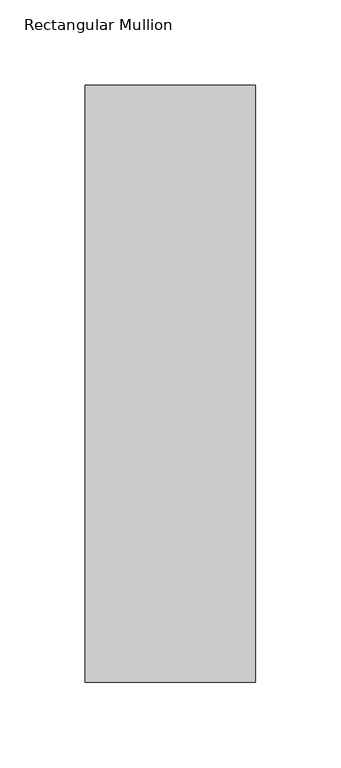
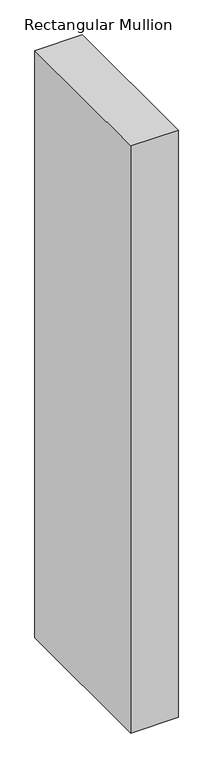
"""IFC4 building model written with IfcOpenShell, lengths in millimetres: member geometry, Rectangular Mullion : WWm-100x350-100mmOffset."""

from ifc_helpers import new_model, si_unit, frame, origin, place, context, project, spatial, polyline, outline, extrude, source, transform, mapped, element, save


def rectangular_mullion_f3706088(model_context):
    return source(origin(), model_context, "Body", "SweptSolid", [
        extrude(outline(polyline([(0.0, 175.0), (0.0, -175.0), (-100.0, -175.0), (-100.0, 175.0), (0.0, 175.0)])), frame((0.0, 0.0, -1310.0), z_axis=(0.0, 0.0, 1.0), x_axis=(1.0, 0.0, 0.0)), (0.0, 0.0, 1.0), 1310.0),
    ])


if __name__ == "__main__":
    model = new_model("IFC4")
    model_context = context("Model", 3, world=origin())
    ifc_project = project(units=[si_unit("LENGTHUNIT", "METRE", prefix="MILLI")], contexts=[model_context])
    site = spatial("IfcSite", under=ifc_project)
    building = spatial("IfcBuilding", under=site)
    placement = place(None, origin())
    rectangular_mullion_shape = rectangular_mullion_f3706088(model_context)
    element("IfcMember", 1, ObjectType="Rectangular Mullion : WWm-100x350-100mmOffset", at=placement, inside=building, context=model_context, shape_type="MappedRepresentation", body=[
        mapped(rectangular_mullion_shape, transform((0.0, 0.0, 0.0), x_axis=(1.0, 0.0, 0.0), y_axis=(0.0, 1.0, 0.0), z_axis=(0.0, 0.0, 1.0))),
    ])
    save(model, "model.ifc")

# Revit data of these elements
# Type "Rectangular Mullion : WWm-100x350-100mmOffset"
#   built-in parameter 1007304 = 1.14829 (stored number, unit not read)
#   built-in parameter 1007301 = 0.164042 (stored number, unit not read)
#   built-in parameter 1007300 = 0.164042 (stored number, unit not read)
# Element 1 (IfcMember, "Rectangular Mullion : WWm-100x350-100mmOffset")
#   Materials on its faces: "WW-EC-RGB-Mullion"
# Materials
#   "WW-EC-RGB-Mullion": class "Generic", colour RGB 255 255 255, transparency 0, Comments = "If region requests black mullions, switch asset color to RGB 25-25-25", Description = "Generic Color", Cost = 0
